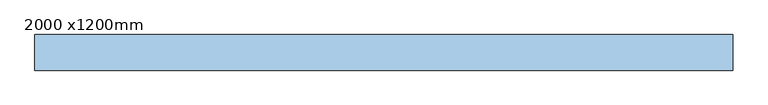
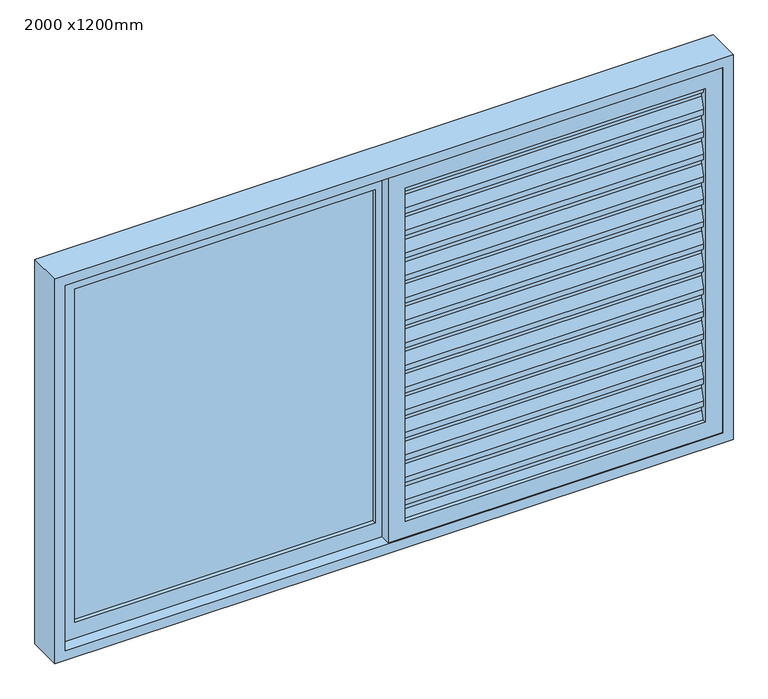
"""IFC4 building model written with IfcOpenShell, lengths in millimetres: window geometry, Janela Veneziana de Correr - 3 Folhas : 2000 x1200mm."""

from ifc_helpers import new_model, si_unit, frame, origin, place, context, project, spatial, polyline, outline, extrude, source, transform, mapped, element, save


def window_2000_x1200mm_dbfbffcb(model_context):
    return source(origin(), model_context, "Body", "SweptSolid", [
        extrude(outline(polyline([(0.6, 1125.0), (0.6, 1105.0), (-6.5028414, 1080.1400549), (-7.5428571, 1080.1400549), (-0.4, 1105.1400549), (-0.4, 1124.0), (-10.4, 1124.0), (-10.4, 1140.1400549), (-0.4, 1175.1400549), (-0.4, 1194.0), (-10.4, 1194.0), (-10.4, 1210.1400549), (-0.4, 1245.1400549), (-0.4, 1264.0), (-10.4, 1264.0), (-10.4, 1280.1400549), (-0.4, 1315.1400549), (-0.4, 1334.0), (-10.4, 1334.0), (-10.4, 1350.1400549), (-0.4, 1385.1400549), (-0.4, 1404.0), (-10.4, 1404.0), (-10.4, 1420.1400549), (-0.4, 1455.1400549), (-0.4, 1474.0), (-10.4, 1474.0), (-10.4, 1490.1400549), (-0.4, 1525.1400549), (-0.4, 1544.0), (-10.4, 1544.0), (-10.4, 1560.1400549), (-0.4, 1595.1400549), (-0.4, 1614.0), (-10.4, 1614.0), (-10.4, 1630.1400549), (-0.4, 1665.1400549), (-0.4, 1684.0), (-10.4, 1684.0), (-10.4, 1700.1400549), (-0.4, 1735.1400549), (-0.4, 1754.0), (-10.4, 1754.0), (-10.4, 1770.1400549), (-0.4, 1805.1400549), (-0.4, 1824.0), (-10.4, 1824.0), (-10.4, 1840.1400549), (-0.4, 1875.1400549), (-0.4, 1894.0), (-10.4, 1894.0), (-10.4, 1910.1400549), (-0.4, 1945.1400549), (-0.4, 1964.0), (-10.4, 1964.0), (-10.4, 1980.1400549), (-0.4, 2015.1400549), (-0.4, 2034.0), (-10.4, 2034.0), (-10.4, 2050.1400549), (-0.4, 2085.1400549), (-0.4, 2104.0), (-10.4, 2104.0), (-10.4, 2120.1400549), (-9.4, 2120.0), (-9.4, 2105.0), (0.6, 2105.0), (0.6, 2085.0), (-9.4, 2050.0), (-9.4, 2035.0), (0.6, 2035.0), (0.6, 2015.0), (-9.4, 1980.0), (-9.4, 1965.0), (0.6, 1965.0), (0.6, 1945.0), (-9.4, 1910.0), (-9.4, 1895.0), (0.6, 1895.0), (0.6, 1875.0), (-9.4, 1840.0), (-9.4, 1825.0), (0.6, 1825.0), (0.6, 1805.0), (-9.4, 1770.0), (-9.4, 1755.0), (0.6, 1755.0), (0.6, 1735.0), (-9.4, 1700.0), (-9.4, 1685.0), (0.6, 1685.0), (0.6, 1665.0), (-9.4, 1630.0), (-9.4, 1615.0), (0.6, 1615.0), (0.6, 1595.0), (-9.4, 1560.0), (-9.4, 1545.0), (0.6, 1545.0), (0.6, 1525.0), (-9.4, 1490.0), (-9.4, 1475.0), (0.6, 1475.0), (0.6, 1455.0), (-9.4, 1420.0), (-9.4, 1405.0), (0.6, 1405.0), (0.6, 1385.0), (-9.4, 1350.0), (-9.4, 1335.0), (0.6, 1335.0), (0.6, 1315.0), (-9.4, 1280.0), (-9.4, 1265.0), (0.6, 1265.0), (0.6, 1245.0), (-9.4, 1210.0), (-9.4, 1195.0), (0.6, 1195.0), (0.6, 1175.0), (-9.4, 1140.0), (-9.4, 1125.0), (0.6, 1125.0)])), frame((35.0, 0.0, 0.0), z_axis=(1.0, 0.0, 0.0), x_axis=(0.0, 1.0, 0.0)), (0.0, 0.0, 1.0), 965.0),
        extrude(outline(polyline([(66.6, 1125.0), (66.6, 1105.0), (59.4971586, 1080.1400549), (58.4571429, 1080.1400549), (65.6, 1105.1400549), (65.6, 1124.0), (55.6, 1124.0), (55.6, 1140.1400549), (65.6, 1175.1400549), (65.6, 1194.0), (55.6, 1194.0), (55.6, 1210.1400549), (65.6, 1245.1400549), (65.6, 1264.0), (55.6, 1264.0), (55.6, 1280.1400549), (65.6, 1315.1400549), (65.6, 1334.0), (55.6, 1334.0), (55.6, 1350.1400549), (65.6, 1385.1400549), (65.6, 1404.0), (55.6, 1404.0), (55.6, 1420.1400549), (65.6, 1455.1400549), (65.6, 1474.0), (55.6, 1474.0), (55.6, 1490.1400549), (65.6, 1525.1400549), (65.6, 1544.0), (55.6, 1544.0), (55.6, 1560.1400549), (65.6, 1595.1400549), (65.6, 1614.0), (55.6, 1614.0), (55.6, 1630.1400549), (65.6, 1665.1400549), (65.6, 1684.0), (55.6, 1684.0), (55.6, 1700.1400549), (65.6, 1735.1400549), (65.6, 1754.0), (55.6, 1754.0), (55.6, 1770.1400549), (65.6, 1805.1400549), (65.6, 1824.0), (55.6, 1824.0), (55.6, 1840.1400549), (65.6, 1875.1400549), (65.6, 1894.0), (55.6, 1894.0), (55.6, 1910.1400549), (65.6, 1945.1400549), (65.6, 1964.0), (55.6, 1964.0), (55.6, 1980.1400549), (65.6, 2015.1400549), (65.6, 2034.0), (55.6, 2034.0), (55.6, 2050.1400549), (65.6, 2085.1400549), (65.6, 2104.0), (55.6, 2104.0), (55.6, 2120.1400549), (56.6, 2120.0), (56.6, 2105.0), (66.6, 2105.0), (66.6, 2085.0), (56.6, 2050.0), (56.6, 2035.0), (66.6, 2035.0), (66.6, 2015.0), (56.6, 1980.0), (56.6, 1965.0), (66.6, 1965.0), (66.6, 1945.0), (56.6, 1910.0), (56.6, 1895.0), (66.6, 1895.0), (66.6, 1875.0), (56.6, 1840.0), (56.6, 1825.0), (66.6, 1825.0), (66.6, 1805.0), (56.6, 1770.0), (56.6, 1755.0), (66.6, 1755.0), (66.6, 1735.0), (56.6, 1700.0), (56.6, 1685.0), (66.6, 1685.0), (66.6, 1665.0), (56.6, 1630.0), (56.6, 1615.0), (66.6, 1615.0), (66.6, 1595.0), (56.6, 1560.0), (56.6, 1545.0), (66.6, 1545.0), (66.6, 1525.0), (56.6, 1490.0), (56.6, 1475.0), (66.6, 1475.0), (66.6, 1455.0), (56.6, 1420.0), (56.6, 1405.0), (66.6, 1405.0), (66.6, 1385.0), (56.6, 1350.0), (56.6, 1335.0), (66.6, 1335.0), (66.6, 1315.0), (56.6, 1280.0), (56.6, 1265.0), (66.6, 1265.0), (66.6, 1245.0), (56.6, 1210.0), (56.6, 1195.0), (66.6, 1195.0), (66.6, 1175.0), (56.6, 1140.0), (56.6, 1125.0), (66.6, 1125.0)])), frame((35.0, 0.0, 0.0), z_axis=(1.0, 0.0, 0.0), x_axis=(0.0, 1.0, 0.0)), (0.0, 0.0, 1.0), 965.0),
        extrude(outline(polyline([(2170.0, -15.0), (1030.0, -15.0), (1030.0, 970.0), (2170.0, 970.0), (2170.0, -15.0)]), holes=[polyline([(2120.0, 35.0), (2120.0, 920.0), (1080.0, 920.0), (1080.0, 35.0), (2120.0, 35.0)])]), frame((0.0, -19.4, 0.0), z_axis=(0.0, 1.0, 0.0), x_axis=(0.0, 0.0, 1.0)), (0.0, 0.0, 1.0), 30.0),
        extrude(outline(polyline([(2170.0, -15.0), (1030.0, -15.0), (1030.0, 970.0), (2170.0, 970.0), (2170.0, -15.0)]), holes=[polyline([(2120.0, 35.0), (2120.0, 920.0), (1080.0, 920.0), (1080.0, 35.0), (2120.0, 35.0)])]), frame((0.0, 46.6, 0.0), z_axis=(0.0, 1.0, 0.0), x_axis=(0.0, 0.0, 1.0)), (0.0, 0.0, 1.0), 30.0),
        extrude(outline(polyline([(-920.0, 25.1), (-920.0, 32.1), (-35.0, 32.1), (-35.0, 25.1), (-920.0, 25.1)])), frame((0.0, 0.0, 1080.0), z_axis=(0.0, 0.0, 1.0), x_axis=(1.0, 0.0, 0.0)), (0.0, 0.0, 1.0), 1040.0),
        extrude(outline(polyline([(2170.0, 15.0), (2170.0, -970.0), (1030.0, -970.0), (1030.0, 15.0), (2170.0, 15.0)]), holes=[polyline([(2120.0, -35.0), (1080.0, -35.0), (1080.0, -920.0), (2120.0, -920.0), (2120.0, -35.0)])]), frame((0.0, 13.6, 0.0), z_axis=(0.0, 1.0, 0.0), x_axis=(0.0, 0.0, 1.0)), (0.0, 0.0, 1.0), 30.0),
        extrude(outline(polyline([(2200.0, 1000.0), (2200.0, -1000.0), (1000.0, -1000.0), (1000.0, 1000.0), (2200.0, 1000.0)]), holes=[polyline([(2170.0, 970.0), (1030.0, 970.0), (1030.0, -970.0), (2170.0, -970.0), (2170.0, 970.0)])]), frame((0.0, -22.4, 0.0), z_axis=(0.0, 1.0, 0.0), x_axis=(0.0, 0.0, 1.0)), (0.0, 0.0, 1.0), 102.0),
    ])


if __name__ == "__main__":
    model = new_model("IFC4")
    model_context = context("Model", 3, world=origin())
    ifc_project = project(units=[si_unit("LENGTHUNIT", "METRE", prefix="MILLI")], contexts=[model_context])
    site = spatial("IfcSite", under=ifc_project)
    building = spatial("IfcBuilding", under=site)
    placement = place(None, origin())
    window_2000_x1200mm_shape = window_2000_x1200mm_dbfbffcb(model_context)
    element("IfcWindow", 1, ObjectType="Janela Veneziana de Correr - 3 Folhas : 2000 x1200mm", at=placement, inside=building, context=model_context, shape_type="MappedRepresentation", body=[
        mapped(window_2000_x1200mm_shape, transform((0.0, 0.0, 0.0), x_axis=(1.0, 0.0, 0.0), y_axis=(0.0, 1.0, 0.0), z_axis=(0.0, 0.0, 1.0))),
    ])
    save(model, "model.ifc")

# Revit data of these elements
# Type "Janela Veneziana de Correr - 3 Folhas : 2000 x1200mm"
#   Type Mark = "J13"
#   SINAPI = ""
#   Tolerância = 0.003 m
#   Módulo Básico M = 0.10 m
#   Largura de Coordenação Modular CM = 2.00 m
#   Largura Vão = 0.965 m
#   Largura Veneziana = 1.00 m
#   Espessura Montante = 0.03 m
#   Largura Batente = 0.10 m
#   L_est_v marco = 0.05 m
#   L_est_h_marco = 0.05 m
#   L_contramarco = 0.03 m
#   Altura de Coordenação Modular CM = 1.20 m
#   Altura Peitoril = 0.95 m
#   Height = 1.20 m
#   Width = 2.00 m
#   Número de Módulos Básicos nM Largura = 20
#   Número de Módulos Básicos nM Altura = 12
#   Material estrutura = Metal - Alumínio
#   Material Quadro = Metal - Alumínio
#   Material Painel = Vidro
#   Type Comments = ""
#   Wall Closure = (empty or 0)
#   Construction Type = (empty or 0)
#   Assembly Code = ""
# Element 1 (IfcWindow, "Janela Veneziana de Correr - 3 Folhas : 2000 x1200mm")
#   Materials on its faces: "Metal - Alumínio", "Vidro"
# Materials
#   "Metal - Alumínio": class "Metal", colour RGB 244 244 244, transparency 0
#   "Vidro": class "Vidro", colour RGB 0 128 192, transparency 0.9, Description = "Vidro de sílica", Cost = 0
